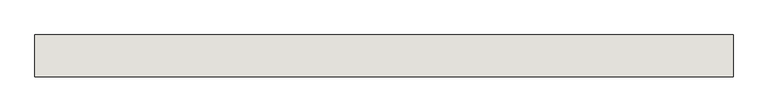
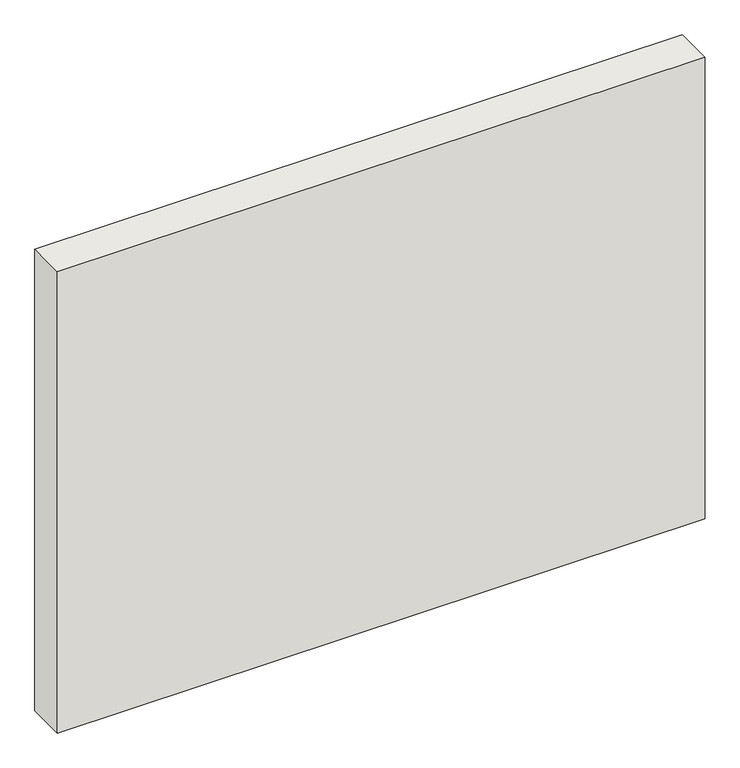
"""IFC4 building model written with IfcOpenShell, lengths in millimetres: wall geometry, Holzwand."""

from ifc_helpers import new_model, si_unit, origin, origin_with_axes, place, context, project, spatial, polyline, outline, extrude, source, transform, mapped, element, save


def wall_187cc882(model_context):
    return source(origin(), model_context, "Body", "SweptSolid", [
        extrude(outline(polyline([(3320.0, 200.0), (3320.0, 0.0), (0.0, 0.0), (0.0, 200.0), (3320.0, 200.0)])), origin_with_axes(), (0.0, 0.0, 1.0), 2500.0),
    ])


if __name__ == "__main__":
    model = new_model("IFC4")
    model_context = context("Model", 3, world=origin())
    ifc_project = project(units=[si_unit("LENGTHUNIT", "METRE", prefix="MILLI")], contexts=[model_context])
    site = spatial("IfcSite", under=ifc_project)
    building = spatial("IfcBuilding", under=site)
    placement = place(None, origin())
    wall_shape = wall_187cc882(model_context)
    element("IfcWall", 1, ObjectType="Holzwand", at=placement, inside=building, context=model_context, shape_type="MappedRepresentation", body=[
        mapped(wall_shape, transform((0.0, 0.0, 0.0), x_axis=(1.0, 0.0, 0.0), y_axis=(0.0, 1.0, 0.0), z_axis=(0.0, 0.0, 1.0))),
    ])
    save(model, "model.ifc")

# Revit data of these elements
# Element 1 (IfcWall, "Holzwand")
#   Materials on its faces: "holzschalung"
# Materials
#   "holzschalung": class "Unassigned", colour RGB 128 128 128, transparency 0
